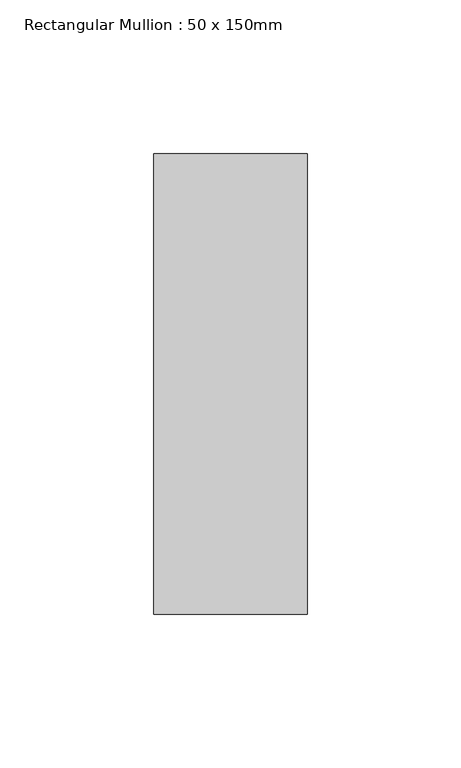
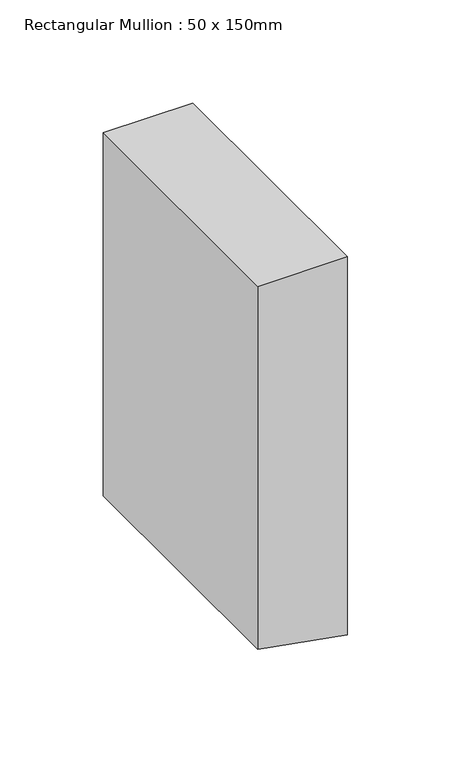
"""IFC4 building model written with IfcOpenShell, lengths in millimetres: member geometry, Rectangular Mullion : 50 x 150mm."""

from ifc_helpers import new_model, si_unit, frame, origin, place, context, project, spatial, polyline, outline, extrude, source, transform, mapped, element, save


def rectangular_mullion_50_x_150mm_e37662f2(model_context):
    return source(origin(), model_context, "Body", "SweptSolid", [
        extrude(outline(polyline([(0.0, 25.0), (0.0, -25.0), (-214.8982375, -25.0), (-220.0718835, 4.3412044), (-223.7145866, 25.0), (0.0, 25.0)])), frame((0.0, -75.0, 0.0), z_axis=(0.0, 1.0, 0.0), x_axis=(0.0, 0.0, 1.0)), (0.0, 0.0, 1.0), 150.0),
    ])


if __name__ == "__main__":
    model = new_model("IFC4")
    model_context = context("Model", 3, world=origin())
    ifc_project = project(units=[si_unit("LENGTHUNIT", "METRE", prefix="MILLI")], contexts=[model_context])
    site = spatial("IfcSite", under=ifc_project)
    building = spatial("IfcBuilding", under=site)
    placement = place(None, origin())
    rectangular_mullion_50_x_150mm_shape = rectangular_mullion_50_x_150mm_e37662f2(model_context)
    element("IfcMember", 1, ObjectType="Rectangular Mullion : 50 x 150mm", at=placement, inside=building, context=model_context, shape_type="MappedRepresentation", body=[
        mapped(rectangular_mullion_50_x_150mm_shape, transform((0.0, 0.0, 0.0), x_axis=(1.0, 0.0, 0.0), y_axis=(0.0, 1.0, 0.0), z_axis=(0.0, 0.0, 1.0))),
    ])
    save(model, "model.ifc")

# Revit data of these elements
# Type "Rectangular Mullion : 50 x 150mm"
#   built-in parameter 1007304 = 0.492126 (stored number, unit not read)
#   built-in parameter 1007301 = 0.082021 (stored number, unit not read)
#   built-in parameter 1007300 = 0.082021 (stored number, unit not read)
# Element 1 (IfcMember, "Rectangular Mullion : 50 x 150mm")
#   Materials on its faces: "Aluminium"
# Materials
#   "Aluminium": class "Metal", colour RGB 247 247 247, transparency 0, Description = "Aluminium 6061", Cost = 0
